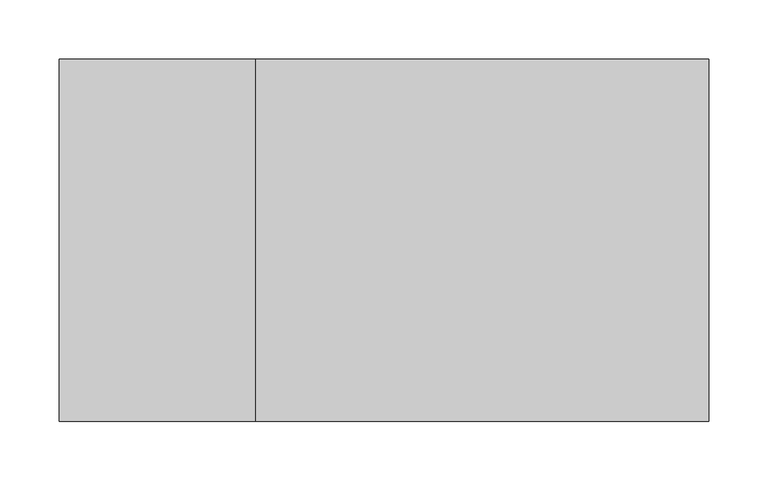
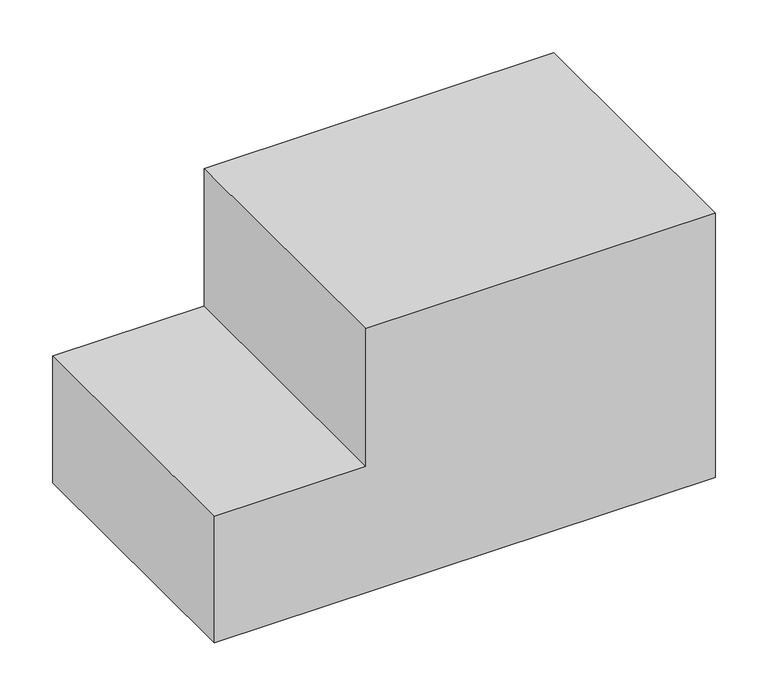
"""IFC4 building model written with IfcOpenShell, lengths in millimetres: proxy geometry, Generic Models 245:Generic Models 245:154686 : Generic Models 245:Generic Models 245:154686."""

from ifc_helpers import new_model, si_unit, frame, origin, place, context, project, spatial, polyline, outline, extrude, source, transform, mapped, element, save


def generic_models_34dbce27(model_context):
    return source(origin(), model_context, "Body", "SweptSolid", [
        extrude(outline(polyline([(139.7, 1850.903213), (139.7, 1685.803213), (-6.35, 1685.803213), (-6.35, 2231.903213), (298.45, 2231.903213), (298.45, 1850.903213), (139.7, 1850.903213)])), frame((0.0, 4450.212823, 0.0), z_axis=(0.0, 1.0, 0.0), x_axis=(0.0, 0.0, 1.0)), (0.0, 0.0, 1.0), 304.8),
    ])


if __name__ == "__main__":
    model = new_model("IFC4")
    model_context = context("Model", 3, world=origin())
    ifc_project = project(units=[si_unit("LENGTHUNIT", "METRE", prefix="MILLI")], contexts=[model_context])
    site = spatial("IfcSite", under=ifc_project)
    building = spatial("IfcBuilding", under=site)
    placement = place(None, origin())
    generic_models_shape = generic_models_34dbce27(model_context)
    element("IfcBuildingElementProxy", 1, Name="Generic Models 245:Generic Models 245:154686 : Generic Models 245:Generic Models 245:154686", ObjectType="Generic Models 245:Generic Models 245:154686 : Generic Models 245:Generic Models 245:154686", at=placement, inside=building, context=model_context, shape_type="MappedRepresentation", body=[
        mapped(generic_models_shape, transform((0.0, 0.0, 0.0), x_axis=(1.0, 0.0, 0.0), y_axis=(0.0, 1.0, 0.0), z_axis=(0.0, 0.0, 1.0))),
    ])
    save(model, "model.ifc")

# Revit data of these elements
# Type "Generic Models 245:Generic Models 245:154686 : Generic Models 245:Generic Models 245:154686"
#   NameOverride = "Generic Models 245:Generic Models 245:154686"
#   ObjectTypeOverride = "Generic Models 245:Generic Models 245"
#   Reference = "Generic Models 245"
#   Category = "Generic Models"
#   Tag = "154686"
# Element 1 (IfcBuildingElementProxy, "Generic Models 245:Generic Models 245:154686 : Generic Models 245:Generic Models 245:154686")
#   Materials on its faces: "_CONCRETE SLAB W/ WIRE MESH (SEE STRUCT. DWGS) - SLOPE 1% AWAY FROM BUILDING 9884"
# Materials
#   "_CONCRETE SLAB W/ WIRE MESH (SEE STRUCT. DWGS) - SLOPE 1% AWAY FROM BUILDING 9884": class "Unassigned", colour RGB 191 191 191, transparency 0
